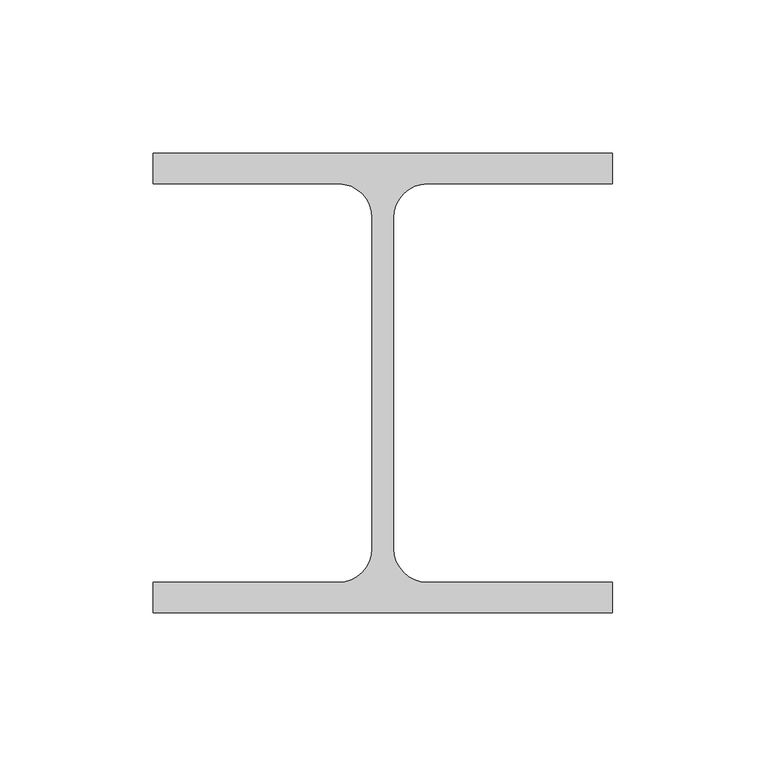
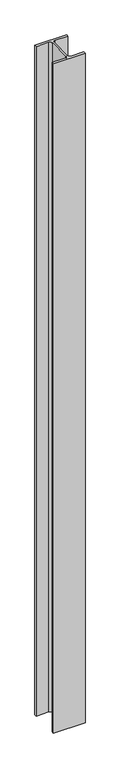
"""IFC4 building model written with IfcOpenShell, lengths in millimetres: column geometry, 0912_Steel Column_H_KSD3502 : H_SC_ASC_H-150x150x7x10."""

from ifc_helpers import new_model, si_unit, point, frame, frame_2d, origin, place, context, project, spatial, polyline, circle_curve, trimmed, segment, composite_curve, outline, extrude, source, transform, mapped, element, save


def column_ee857ed7(model_context):
    return source(origin(), model_context, "Body", "SweptSolid", [
        extrude(outline(composite_curve([segment(polyline([(75.0, 75.0), (75.0, 65.0), (14.5, 65.0)]), True, "CONTINUOUS"), segment(trimmed(circle_curve(frame_2d((14.5, 54.0)), 11.0), [point((14.5, 65.0))], [point((3.5, 54.0))], True, "CARTESIAN"), True, "CONTINUOUS"), segment(polyline([(3.5, 54.0), (3.5, -54.0)]), True, "CONTINUOUS"), segment(trimmed(circle_curve(frame_2d((14.5, -54.0)), 11.0), [point((3.5, -54.0))], [point((14.5, -65.0))], True, "CARTESIAN"), True, "CONTINUOUS"), segment(polyline([(14.5, -65.0), (75.0, -65.0), (75.0, -75.0), (-75.0, -75.0), (-75.0, -65.0), (-14.5, -65.0)]), True, "CONTINUOUS"), segment(trimmed(circle_curve(frame_2d((-14.5, -54.0)), 11.0), [point((-14.5, -65.0))], [point((-3.5, -54.0))], True, "CARTESIAN"), True, "CONTINUOUS"), segment(polyline([(-3.5, -54.0), (-3.5, 54.0)]), True, "CONTINUOUS"), segment(trimmed(circle_curve(frame_2d((-14.5, 54.0)), 11.0), [point((-3.5, 54.0))], [point((-14.5, 65.0))], True, "CARTESIAN"), True, "CONTINUOUS"), segment(polyline([(-14.5, 65.0), (-75.0, 65.0), (-75.0, 75.0), (75.0, 75.0)]), True, "CONTINUOUS")], self_intersect=False)), frame((0.0, 0.0, 4617.9720055), z_axis=(0.0, 0.0, 1.0), x_axis=(1.0, 0.0, 0.0)), (0.0, 0.0, 1.0), 3342.0),
    ])


if __name__ == "__main__":
    model = new_model("IFC4")
    model_context = context("Model", 3, world=origin())
    ifc_project = project(units=[si_unit("LENGTHUNIT", "METRE", prefix="MILLI")], contexts=[model_context])
    site = spatial("IfcSite", under=ifc_project)
    building = spatial("IfcBuilding", under=site)
    placement = place(None, origin())
    column_shape = column_ee857ed7(model_context)
    element("IfcColumn", 1, ObjectType="0912_Steel Column_H_KSD3502 : H_SC_ASC_H-150x150x7x10", at=placement, inside=building, context=model_context, shape_type="MappedRepresentation", body=[
        mapped(column_shape, transform((0.0, 0.0, 0.0), x_axis=(1.0, 0.0, 0.0), y_axis=(0.0, 1.0, 0.0), z_axis=(0.0, 0.0, 1.0))),
    ])
    save(model, "model.ifc")

# Revit data of these elements
# Type "0912_Steel Column_H_KSD3502 : H_SC_ASC_H-150x150x7x10"
#   H_WM Code_1 = "S01AA002-00001 | Main Steel Structure Fabrication Work | Shelter/Building | Medium Steel - Standard (90KG/M>Weight≥30KG/M) | Material: (   )"
#   H_WM Code_2 = "S03AA028-00001 | Main Steel Structure Erection Work | Shelter/Building | Medium Steel (90KG/M>Weight≥30KG/M) | Material: (   )"
#   H_WM Code_3 = "S01AA010-00001 | Main Steel Structure Fabrication Work | Shelter/Building | Steel Painting/Coating | for Non-Fireproofed Steel Surface, Surface Preparation, Primer, Second & Final Coat | Material: (   )"
#   H_Q'ty Cal Type Tag = "SC-Q2"
#   Width = 15.0 cm
#   Web Thickness = 0.7 cm
#   Web Fillet = 1.1 cm
#   Warping Constant = 27562.5 cm⁶
#   Torsional Moment of Inertia = 11.6007 cm⁴
#   Section Area = 40.14 cm²
#   Plastic Modulus weak axis = 115.0 cm³
#   Plastic Modulus strong axis = 246.0 cm³
#   Perimeter = 0.87 m²/m
#   Nominal Weight = 31.50 kgf/m
#   Moment of Inertia weak axis = 563.00 cm⁴
#   Moment of Inertia strong axis = 1640.00 cm⁴
#   Height = 15.0 cm
#   Flange Thickness = 1.0 cm
#   Elastic Modulus weak axis = 75.1 cm³
#   Elastic Modulus strong axis = 219.0 cm³
#   Centroid Vertical = 7.5 cm
#   Centroid Horizontal = 7.5 cm
#   Structural Material [instance default] = Steel, 45-345
#   Section Name Key = ""
#   Bolt Spacing = 0
#   Assembly Code = ""
# Element 1 (IfcColumn, "0912_Steel Column_H_KSD3502 : H_SC_ASC_H-150x150x7x10")
#   Structural Material = none
# Materials
#   "Steel, 45-345": class "Metal", colour RGB 189 187 185, transparency 0, Description = "Steel 345 MPa", Cost = 0
